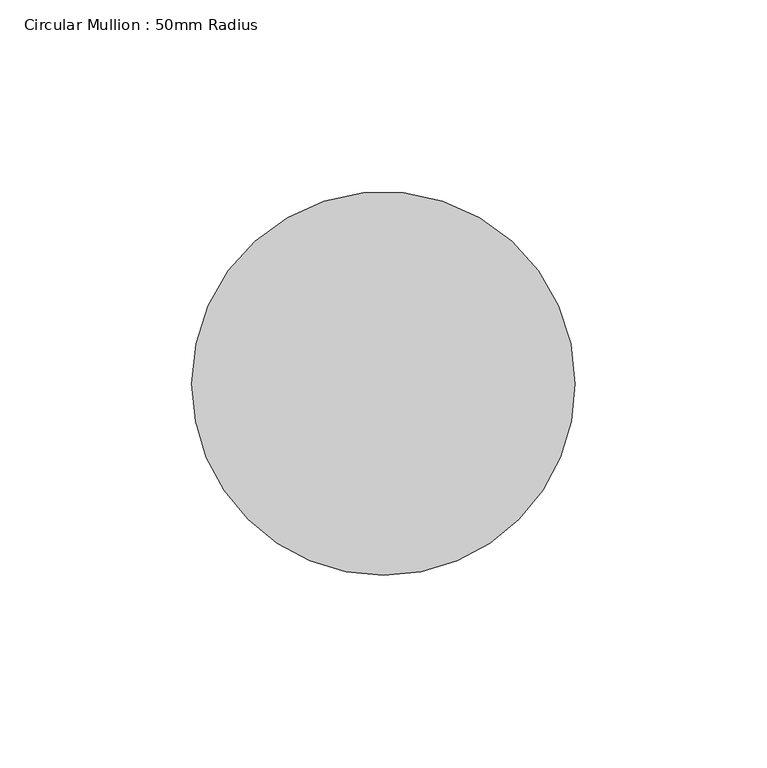
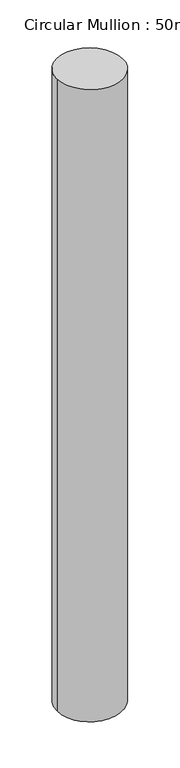
"""IFC4 building model written with IfcOpenShell, lengths in millimetres: member geometry, Circular Mullion : 50mm Radius."""

from ifc_helpers import new_model, si_unit, frame, origin, place, context, project, spatial, ellipse_curve, source, transform, mapped, element, save
from ifc_brep_helpers import plane_surface, cylinder_surface, advanced_brep


def circular_mullion_50mm_radius_882b9640(model_context):
    return source(origin(), model_context, "Body", "AdvancedBrep", [
        advanced_brep(
        [(-100.0, 0.0, 2.2809397), (0.0, 0.0, 0.0), (0.0, 0.0, -1009.164291), (-100.0, 0.0, -1011.417067)],
        [
            (0, 1, ellipse_curve(frame((-50.0, 0.0, 1.1404699), z_axis=(-0.022797920531318495, -0.02205254886478132, -0.9994968433707104), x_axis=(-0.7183973164529182, -0.6949095161395192, 0.03171845034022377)), 50.0251705, 50.0)),
            (1, 2),
            (2, 3, ellipse_curve(frame((-50.0, 0.0, -1010.290679), z_axis=(-0.022516702609528132, -0.021780525284671864, 0.9995091829602758), x_axis=(0.7184061856435722, 0.6949180953543891, 0.0313271955029747)), 50.0245529, 50.0)),
            (3, 0),
            (1, 0, ellipse_curve(frame((-50.0, 0.0, 1.1404699), z_axis=(-0.022797920531318495, -0.02205254886478132, -0.9994968433707104), x_axis=(-0.7183973164529182, -0.6949095161395192, 0.03171845034022377)), 50.0251705, 50.0)),
            (3, 2, ellipse_curve(frame((-50.0, 0.0, -1010.290679), z_axis=(-0.022516702609528132, -0.021780525284671864, 0.9995091829602758), x_axis=(0.7184061856435722, 0.6949180953543891, 0.0313271955029747)), 50.0245529, 50.0)),
        ],
        [
            cylinder_surface(frame((-50.0, 0.0, 0.0), z_axis=(0.0, 0.0, 1.0), x_axis=(1.0, 0.0, 0.0)), 50.0),
            plane_surface(frame((-211.915047, 219.0777325, 0.0), z_axis=(0.022797920531318495, 0.02205254886478132, 0.9994968433707104), x_axis=(0.7183973164529182, 0.6949095161395188, -0.03171845034023386))),
            plane_surface(frame((-211.915047, 219.0777325, -1009.164291), z_axis=(0.022516702609528132, 0.021780525284671864, -0.9995091829602758), x_axis=(0.7184061856435721, 0.6949180953543888, 0.031327195502983685))),
        ],
        [
            (0, [[1, 2, 3, 4]]),
            (0, [[5, -4, 6, -2]]),
            (1, [[-1, -5]]),
            (2, [[-6, -3]]),
        ],
    ),
    ])


if __name__ == "__main__":
    model = new_model("IFC4")
    model_context = context("Model", 3, world=origin())
    ifc_project = project(units=[si_unit("LENGTHUNIT", "METRE", prefix="MILLI")], contexts=[model_context])
    site = spatial("IfcSite", under=ifc_project)
    building = spatial("IfcBuilding", under=site)
    placement = place(None, origin())
    circular_mullion_50mm_radius_shape = circular_mullion_50mm_radius_882b9640(model_context)
    element("IfcMember", 1, ObjectType="Circular Mullion : 50mm Radius", at=placement, inside=building, context=model_context, shape_type="MappedRepresentation", body=[
        mapped(circular_mullion_50mm_radius_shape, transform((0.0, 0.0, 0.0), x_axis=(1.0, 0.0, 0.0), y_axis=(0.0, 1.0, 0.0), z_axis=(0.0, 0.0, 1.0))),
    ])
    save(model, "model.ifc")

# Revit data of these elements
# Type "Circular Mullion : 50mm Radius"
#   built-in parameter 1007350 = 0.164042 (stored number, unit not read)
# Element 1 (IfcMember, "Circular Mullion : 50mm Radius")
#   Materials on its faces: "Aluminium"
# Materials
#   "Aluminium": class "Metal", colour RGB 247 247 247, transparency 0, Description = "Aluminium 6061", Cost = 0
